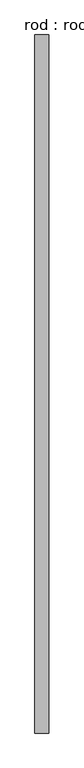
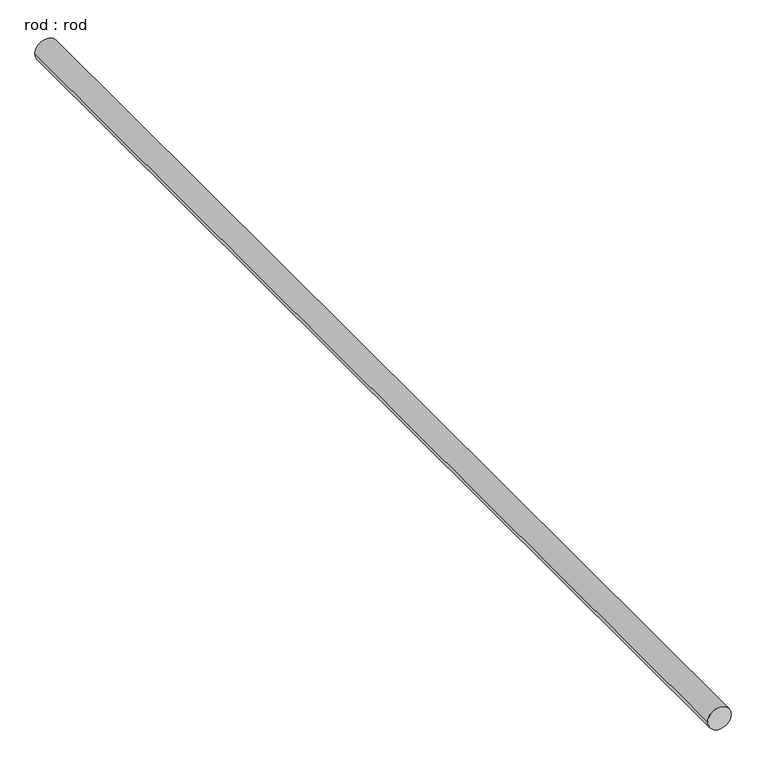
"""IFC4 building model written with IfcOpenShell, lengths in millimetres: proxy geometry, rod : rod."""

import ifcopenshell
import ifcopenshell.guid

model = None  # the IFC model being written
_history = None  # IfcOwnerHistory: only IFC2X3 demands one
_inside = {}  # id of a spatial element -> (the spatial element, [elements in it])
_under = {}  # id of a project, library or spatial element -> (it, [spatial elements below it])
_declared = {}  # id of a project -> (the project, [libraries it declares])
_typed = {}  # id of a type object -> (the type object, [elements of that type])
_made_of = {}  # id of a material, layer set ... -> (it, [elements and type objects made of it])


def new_model(schema):
    """Start an empty IFC model of exactly this schema.

    Asked for "IFC4X3", IfcOpenShell would pick the latest addendum, in which some entities
    have other attributes; the version numbers below select the first issue.
    IFC2X3 requires an IfcOwnerHistory on every rooted entity: one is made here for all.
    """
    global model, _history
    if schema == "IFC4X3":
        model = ifcopenshell.file(schema_version=(4, 3, 0, 0))
    else:
        model = ifcopenshell.file(schema=schema)
    _inside.clear()
    _under.clear()
    _declared.clear()
    _typed.clear()
    _made_of.clear()
    _history = None
    if model.schema == "IFC2X3":
        org = make("IfcOrganization", Name="unknown")
        user = make(
            "IfcPersonAndOrganization",
            ThePerson=make("IfcPerson", FamilyName="unknown"),
            TheOrganization=org,
        )
        app = make(
            "IfcApplication",
            ApplicationDeveloper=org,
            Version="unknown",
            ApplicationFullName="unknown",
            ApplicationIdentifier="unknown",
        )
        _history = make(
            "IfcOwnerHistory",
            OwningUser=user,
            OwningApplication=app,
            ChangeAction="ADDED",
            CreationDate=0,
        )
    return model


def make(cls, **values):
    """One entity of the class cls with the attributes given. An attribute that is None is left unset."""
    return model.create_entity(
        cls, **{name: value for name, value in values.items() if value is not None}
    )


def rooted(cls, **values):
    """An entity with a GlobalId (a new one), such as an element, a storey or a relation."""
    return make(cls, GlobalId=ifcopenshell.guid.new(), OwnerHistory=_history, **values)


def si_unit(unit_type, name, prefix=None):
    """IfcSIUnit, for example si_unit("LENGTHUNIT", "METRE", prefix="MILLI")."""
    return make("IfcSIUnit", UnitType=unit_type, Prefix=prefix, Name=name)


def assignment(units):
    """IfcUnitAssignment: the units of a project."""
    return None if units is None else make("IfcUnitAssignment", Units=units)


def point(xyz):
    """IfcCartesianPoint."""
    return None if xyz is None else make("IfcCartesianPoint", Coordinates=xyz)


def direction(xyz):
    """IfcDirection."""
    return None if xyz is None else make("IfcDirection", DirectionRatios=xyz)


def frame(location, z_axis=None, x_axis=None):
    """IfcAxis2Placement3D, a coordinate frame: its origin and axes. An axis left out is left unset."""
    return make(
        "IfcAxis2Placement3D",
        Location=point(location),
        Axis=direction(z_axis),
        RefDirection=direction(x_axis),
    )


def frame_2d(location, x_axis=None):
    """IfcAxis2Placement2D, a coordinate frame in the plane: its origin and x axis."""
    return make(
        "IfcAxis2Placement2D", Location=point(location), RefDirection=direction(x_axis)
    )


def origin():
    """The frame at (0, 0, 0) with its axes left unset."""
    return frame((0.0, 0.0, 0.0))


def place(relative_to, where):
    """IfcLocalPlacement: puts the frame where relative to a parent placement (None: the world)."""
    return make(
        "IfcLocalPlacement", PlacementRelTo=relative_to, RelativePlacement=where
    )


def context(
    kind, dimensions, precision=None, world=None, true_north=None, identifier=None
):
    """IfcGeometricRepresentationContext, for example the 3D "Model" context."""
    return make(
        "IfcGeometricRepresentationContext",
        ContextIdentifier=identifier,
        ContextType=kind,
        CoordinateSpaceDimension=dimensions,
        Precision=precision,
        WorldCoordinateSystem=world,
        TrueNorth=true_north,
    )


def project(units=None, contexts=None):
    """IfcProject with its units and contexts."""
    return rooted(
        "IfcProject",
        Name="project",
        RepresentationContexts=contexts,
        UnitsInContext=assignment(units),
    )


def spatial(cls, under=None, at=None, **own):
    """A site, building, storey or space (cls), placed at a placement, below another one or the project."""
    s = rooted(cls, ObjectPlacement=at, **own)
    if under is not None:
        _under.setdefault(under.id(), (under, []))[1].append(s)
    return s


def circle_curve(where, radius):
    """IfcCircle in the frame where."""
    return make("IfcCircle", Position=where, Radius=radius)


def trimmed(basis, trim1, trim2, sense, master):
    """IfcTrimmedCurve: the piece of a basis curve between two trims."""
    return make(
        "IfcTrimmedCurve",
        BasisCurve=basis,
        Trim1=trim1,
        Trim2=trim2,
        SenseAgreement=sense,
        MasterRepresentation=master,
    )


def segment(curve, same_sense, transition):
    """IfcCompositeCurveSegment."""
    return make(
        "IfcCompositeCurveSegment",
        Transition=transition,
        SameSense=same_sense,
        ParentCurve=curve,
    )


def composite_curve(segments, self_intersect=None):
    """IfcCompositeCurve: segments joined end to end."""
    return make("IfcCompositeCurve", Segments=segments, SelfIntersect=self_intersect)


def outline(outer, holes=None, kind="AREA"):
    """IfcArbitraryClosedProfileDef: a profile drawn as a closed curve; with holes, ...WithVoids."""
    if holes is None:
        return make("IfcArbitraryClosedProfileDef", ProfileType=kind, OuterCurve=outer)
    return make(
        "IfcArbitraryProfileDefWithVoids",
        ProfileType=kind,
        OuterCurve=outer,
        InnerCurves=holes,
    )


def extrude(swept, where, along, depth):
    """IfcExtrudedAreaSolid: the profile swept, set in the frame where, extruded along a direction by depth."""
    return make(
        "IfcExtrudedAreaSolid",
        SweptArea=swept,
        Position=where,
        ExtrudedDirection=direction(along),
        Depth=depth,
    )


def shape(context_of_items, identifier, shape_type, items):
    """IfcShapeRepresentation: the items that make up one representation, for example the "Body"."""
    return make(
        "IfcShapeRepresentation",
        ContextOfItems=context_of_items,
        RepresentationIdentifier=identifier,
        RepresentationType=shape_type,
        Items=items,
    )


def source(mapping_origin, context_of_items, identifier, shape_type, items):
    """IfcRepresentationMap: a shape defined once, which mapped items show again and again."""
    return make(
        "IfcRepresentationMap",
        MappingOrigin=mapping_origin,
        MappedRepresentation=shape(context_of_items, identifier, shape_type, items),
    )


def transform(
    local_origin,
    x_axis=None,
    y_axis=None,
    z_axis=None,
    scale=None,
    scale2=None,
    scale3=None,
    uniform=True,
):
    """IfcCartesianTransformationOperator3D, or its non-uniform kind. x_axis, y_axis, z_axis: its Axis1, 2, 3."""
    if uniform:
        return make(
            "IfcCartesianTransformationOperator3D",
            Axis1=direction(x_axis),
            Axis2=direction(y_axis),
            LocalOrigin=point(local_origin),
            Scale=scale,
            Axis3=direction(z_axis),
        )
    return make(
        "IfcCartesianTransformationOperator3DnonUniform",
        Axis1=direction(x_axis),
        Axis2=direction(y_axis),
        LocalOrigin=point(local_origin),
        Scale=scale,
        Axis3=direction(z_axis),
        Scale2=scale2,
        Scale3=scale3,
    )


def mapped(mapping_source, mapping_target):
    """IfcMappedItem: shows the shape of a source again, moved by a transform."""
    return make(
        "IfcMappedItem", MappingSource=mapping_source, MappingTarget=mapping_target
    )


def made_of(thing, what):
    """Note that an element or type object is made of a material, layer set ...; save() writes the relation."""
    if what is not None:
        _made_of.setdefault(what.id(), (what, []))[1].append(thing)
    return thing


def element(
    cls,
    number,
    at=None,
    inside=None,
    cuts=None,
    type_object=None,
    material=None,
    context=None,
    identifier="Body",
    shape_type=None,
    held_by="IfcProductDefinitionShape",
    body=None,
    shapes=None,
    **own,
):
    """One element of the class cls, such as IfcWall. Its Tag is "e" and its number.

    at: its placement. inside: the storey or other place that contains it. cuts: it is an
    opening in that element (IfcRelVoidsElement). A single representation is given by context,
    identifier, shape_type and body (its items); several are given by shapes. held_by: the class
    of the entity that holds the representations. save() writes the other relations.
    """
    e = rooted(cls, Tag="e%d" % number, ObjectPlacement=at, **own)
    if body is not None:
        shapes = [shape(context, identifier, shape_type, body)]
    if shapes is not None:
        e.Representation = make(held_by, Representations=shapes)
    if inside is not None:
        _inside.setdefault(inside.id(), (inside, []))[1].append(e)
    if cuts is not None:
        rooted(
            "IfcRelVoidsElement", RelatingBuildingElement=cuts, RelatedOpeningElement=e
        )
    if type_object is not None:
        _typed.setdefault(type_object.id(), (type_object, []))[1].append(e)
    return made_of(e, material)


def aggregate(whole, parts):
    """IfcRelAggregates: a whole, such as a stair, and the parts it consists of."""
    return rooted("IfcRelAggregates", RelatingObject=whole, RelatedObjects=parts)


def save(model, path):
    """Write the relations noted so far, then the file.

    IfcRelAggregates (storeys below a building ...), IfcRelContainedInSpatialStructure (elements
    in a storey), IfcRelDefinesByType, IfcRelAssociatesMaterial and IfcRelDeclares: one each for
    every whole, place, type object, material and project.
    """
    for whole, parts in _under.values():
        aggregate(whole, parts)
    for where, things in _inside.values():
        rooted(
            "IfcRelContainedInSpatialStructure",
            RelatedElements=things,
            RelatingStructure=where,
        )
    for kind, things in _typed.values():
        rooted("IfcRelDefinesByType", RelatedObjects=things, RelatingType=kind)
    for what, things in _made_of.values():
        rooted("IfcRelAssociatesMaterial", RelatedObjects=things, RelatingMaterial=what)
    for by, libraries in _declared.values():
        rooted("IfcRelDeclares", RelatingContext=by, RelatedDefinitions=libraries)
    model.write(path)


def rod_rod_f8a6c655(model_context):
    return source(origin(), model_context, "Body", "SweptSolid", [
        extrude(outline(composite_curve([segment(trimmed(circle_curve(frame_2d((0.0108462, 0.0)), 200.0), [point((0.0108462, 200.0))], [point((0.0108462, -200.0))], False, "CARTESIAN"), True, "CONTINUOUS"), segment(trimmed(circle_curve(frame_2d((0.0108462, 0.0)), 200.0), [point((0.0108462, -200.0))], [point((0.0108462, 200.0))], False, "CARTESIAN"), True, "CONTINUOUS")], self_intersect=False)), frame((0.0, -5907.2713847, 0.0), z_axis=(0.0, 1.0, 0.0), x_axis=(0.0, 0.0, 1.0)), (0.0, 0.0, 1.0), 20000.0),
    ])


if __name__ == "__main__":
    model = new_model("IFC4")
    model_context = context("Model", 3, world=origin())
    ifc_project = project(units=[si_unit("LENGTHUNIT", "METRE", prefix="MILLI")], contexts=[model_context])
    site = spatial("IfcSite", under=ifc_project)
    building = spatial("IfcBuilding", under=site)
    placement = place(None, origin())
    rod_rod_shape = rod_rod_f8a6c655(model_context)
    element("IfcBuildingElementProxy", 1, Name="rod : rod", ObjectType="rod : rod", at=placement, inside=building, context=model_context, shape_type="MappedRepresentation", body=[
        mapped(rod_rod_shape, transform((0.0, 0.0, 0.0), x_axis=(1.0, 0.0, 0.0), y_axis=(0.0, 1.0, 0.0), z_axis=(0.0, 0.0, 1.0))),
    ])
    save(model, "model.ifc")

# Revit data of these elements
# Type "rod : rod"
#   Default Elevation = 0
